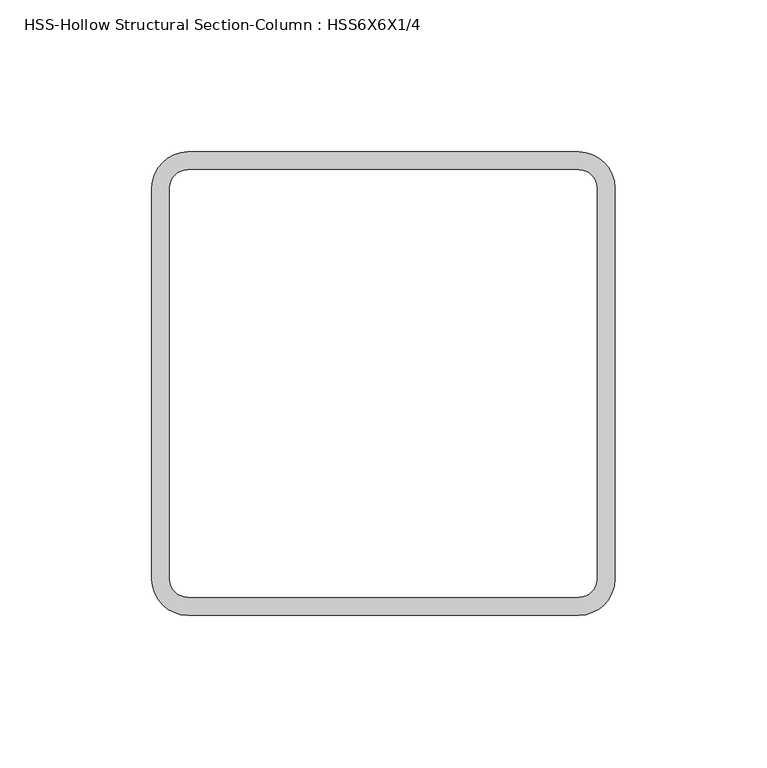
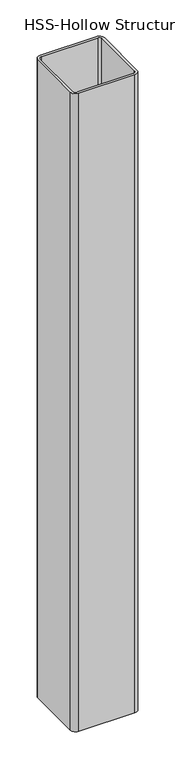
"""IFC4 building model written with IfcOpenShell, lengths in millimetres: column geometry, HSS-Hollow Structural Section-Column : HSS6X6X1/4."""

from ifc_helpers import new_model, si_unit, point, frame, frame_2d, origin, place, context, project, spatial, polyline, circle_curve, trimmed, segment, composite_curve, outline, extrude, source, transform, mapped, element, save


def hss_hollow_structural_section_column_hss6x6x1_4_6d19ae03(model_context):
    return source(origin(), model_context, "Body", "SweptSolid", [
        extrude(outline(composite_curve([segment(trimmed(circle_curve(frame_2d((64.3636, 64.3636)), 11.8364), [point((64.3636, 76.2))], [point((76.2, 64.3636))], False, "CARTESIAN"), True, "CONTINUOUS"), segment(polyline([(76.2, 64.3636), (76.2, -64.3636)]), True, "CONTINUOUS"), segment(trimmed(circle_curve(frame_2d((64.3636, -64.3636)), 11.8364), [point((76.2, -64.3636))], [point((64.3636, -76.2))], False, "CARTESIAN"), True, "CONTINUOUS"), segment(polyline([(64.3636, -76.2), (-64.3636, -76.2)]), True, "CONTINUOUS"), segment(trimmed(circle_curve(frame_2d((-64.3636, -64.3636)), 11.8364), [point((-64.3636, -76.2))], [point((-76.2, -64.3636))], False, "CARTESIAN"), True, "CONTINUOUS"), segment(polyline([(-76.2, -64.3636), (-76.2, 64.3636)]), True, "CONTINUOUS"), segment(trimmed(circle_curve(frame_2d((-64.3636, 64.3636)), 11.8364), [point((-76.2, 64.3636))], [point((-64.3636, 76.2))], False, "CARTESIAN"), True, "CONTINUOUS"), segment(polyline([(-64.3636, 76.2), (64.3636, 76.2)]), True, "CONTINUOUS")], self_intersect=False), holes=[composite_curve([segment(polyline([(64.3636, 70.2818), (-64.3636, 70.2818)]), True, "CONTINUOUS"), segment(trimmed(circle_curve(frame_2d((-64.3636, 64.3636)), 5.9182), [point((-64.3636, 70.2818))], [point((-70.2818, 64.3636))], True, "CARTESIAN"), True, "CONTINUOUS"), segment(polyline([(-70.2818, 64.3636), (-70.2818, -64.3636)]), True, "CONTINUOUS"), segment(trimmed(circle_curve(frame_2d((-64.3636, -64.3636)), 5.9182), [point((-70.2818, -64.3636))], [point((-64.3636, -70.2818))], True, "CARTESIAN"), True, "CONTINUOUS"), segment(polyline([(-64.3636, -70.2818), (64.3636, -70.2818)]), True, "CONTINUOUS"), segment(trimmed(circle_curve(frame_2d((64.3636, -64.3636)), 5.9182), [point((64.3636, -70.2818))], [point((70.2818, -64.3636))], True, "CARTESIAN"), True, "CONTINUOUS"), segment(polyline([(70.2818, -64.3636), (70.2818, 64.3636)]), True, "CONTINUOUS"), segment(trimmed(circle_curve(frame_2d((64.3636, 64.3636)), 5.9182), [point((70.2818, 64.3636))], [point((64.3636, 70.2818))], True, "CARTESIAN"), True, "CONTINUOUS")], self_intersect=False)]), frame((0.0, 0.0, 27787.6), z_axis=(0.0, 0.0, 1.0), x_axis=(1.0, 0.0, 0.0)), (0.0, 0.0, 1.0), 1543.05),
    ])


if __name__ == "__main__":
    model = new_model("IFC4")
    model_context = context("Model", 3, world=origin())
    ifc_project = project(units=[si_unit("LENGTHUNIT", "METRE", prefix="MILLI")], contexts=[model_context])
    site = spatial("IfcSite", under=ifc_project)
    building = spatial("IfcBuilding", under=site)
    placement = place(None, origin())
    hss_hollow_structural_section_column_hss6x6x1_4_shape = hss_hollow_structural_section_column_hss6x6x1_4_6d19ae03(model_context)
    element("IfcColumn", 1, ObjectType="HSS-Hollow Structural Section-Column : HSS6X6X1/4", at=placement, inside=building, context=model_context, shape_type="MappedRepresentation", body=[
        mapped(hss_hollow_structural_section_column_hss6x6x1_4_shape, transform((0.0, 0.0, 0.0), x_axis=(1.0, 0.0, 0.0), y_axis=(0.0, 1.0, 0.0), z_axis=(0.0, 0.0, 1.0))),
    ])
    save(model, "model.ifc")

# Revit data of these elements
# Type "HSS-Hollow Structural Section-Column : HSS6X6X1/4"
#   Assembly Code = "B10"
#   Shape = "Square"
#   W = 19
#   Ht = 0' - 6"
#   b = 0' - 6"
#   kr = 0' - 0.466"
#   t = 0' - 0.233"
#   A = 0.0363889 SF
#   Structural Material [instance default] = Steel ASTM A500, Grade B, Rectangular and Square
# Element 1 (IfcColumn, "HSS-Hollow Structural Section-Column : HSS6X6X1/4")
#   Materials on its faces: "Steel ASTM A500, Grade B, Rectangular and Square"
# Materials
#   "Steel ASTM A500, Grade B, Rectangular and Square": class "Metal", colour RGB 199 199 199, transparency 0, Description = "Carbon steel", Cost = 0
